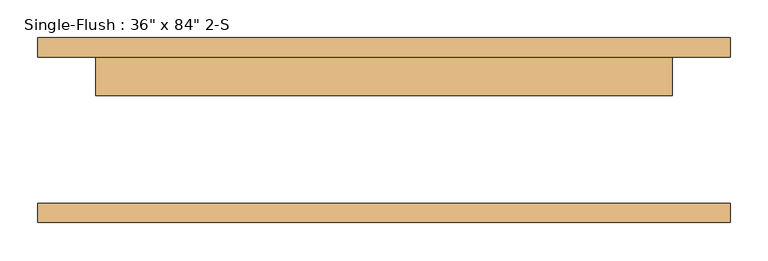
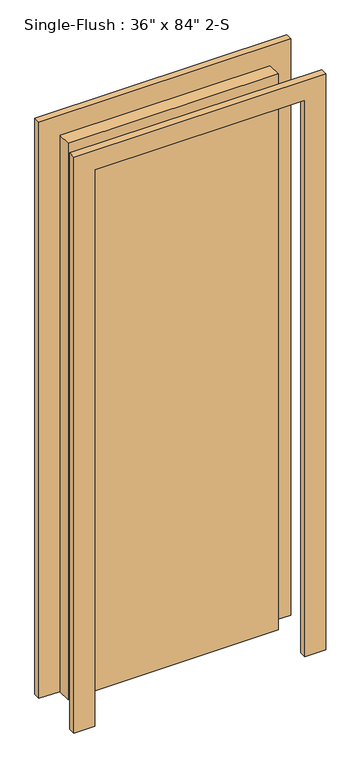
"""IFC4 building model written with IfcOpenShell, lengths in millimetres: door geometry."""

from ifc_helpers import new_model, si_unit, frame, origin, origin_with_axes, place, context, project, spatial, polyline, outline, extrude, source, transform, mapped, element, save


def door_4d1dec4c(model_context):
    return source(origin(), model_context, "Body", "SweptSolid", [
        extrude(outline(polyline([(2209.8, -457.2), (0.0, -457.2), (0.0, -381.0), (2133.6, -381.0), (2133.6, 381.0), (0.0, 381.0), (0.0, 457.2), (2209.8, 457.2), (2209.8, -457.2)])), frame((0.0, 96.8375, 0.0), z_axis=(0.0, 1.0, 0.0), x_axis=(0.0, 0.0, 1.0)), (0.0, 0.0, 1.0), 25.4),
        extrude(outline(polyline([(2209.8, 457.2), (2209.8, -457.2), (0.0, -457.2), (0.0, -381.0), (2133.6, -381.0), (2133.6, 381.0), (0.0, 381.0), (0.0, 457.2), (2209.8, 457.2)])), frame((0.0, -122.2375, 0.0), z_axis=(0.0, 1.0, 0.0), x_axis=(0.0, 0.0, 1.0)), (0.0, 0.0, 1.0), 25.4),
        extrude(outline(polyline([(381.0, 46.0375), (-381.0, 46.0375), (-381.0, 96.8375), (381.0, 96.8375), (381.0, 46.0375)])), origin_with_axes(), (0.0, 0.0, 1.0), 2133.6),
    ])


if __name__ == "__main__":
    model = new_model("IFC4")
    model_context = context("Model", 3, world=origin())
    ifc_project = project(units=[si_unit("LENGTHUNIT", "METRE", prefix="MILLI")], contexts=[model_context])
    site = spatial("IfcSite", under=ifc_project)
    building = spatial("IfcBuilding", under=site)
    placement = place(None, origin())
    door_shape = door_4d1dec4c(model_context)
    element("IfcDoor", 1, ObjectType="Single-Flush : 36\" x 84\" 2-S", at=placement, inside=building, context=model_context, shape_type="MappedRepresentation", body=[
        mapped(door_shape, transform((0.0, 0.0, 0.0), x_axis=(1.0, 0.0, 0.0), y_axis=(0.0, 1.0, 0.0), z_axis=(0.0, 0.0, 1.0))),
    ])
    save(model, "model.ifc")

# Revit data of these elements
# Type "Single-Flush : 36\" x 84\" 2-S"
#   Type Mark = "57"
#   Assembly Code = "C1020"
#   Thickness = 0' - 2"
#   Height = 7' - 0"
#   Trim Projection Ext = 0' - 1"
#   Trim Projection Int = 0' - 1"
#   Trim Width = 0' - 3"
#   Width = 2' - 6"
#   Door Material = Door - Panel
#   Frame Material = Door - Frame
#   Wall Closure = (empty or 0)
# Element 1 (IfcDoor, "Single-Flush : 36\" x 84\" 2-S")
#   Materials on its faces: "Door - Frame", "Door - Panel"
# Materials
#   "Door - Panel": class "Wood", colour RGB 227 170 128, transparency 0, Cost = 0
#   "Door - Frame": class "Miscellaneous", colour RGB 153 76 43, transparency 0, Cost = 0
